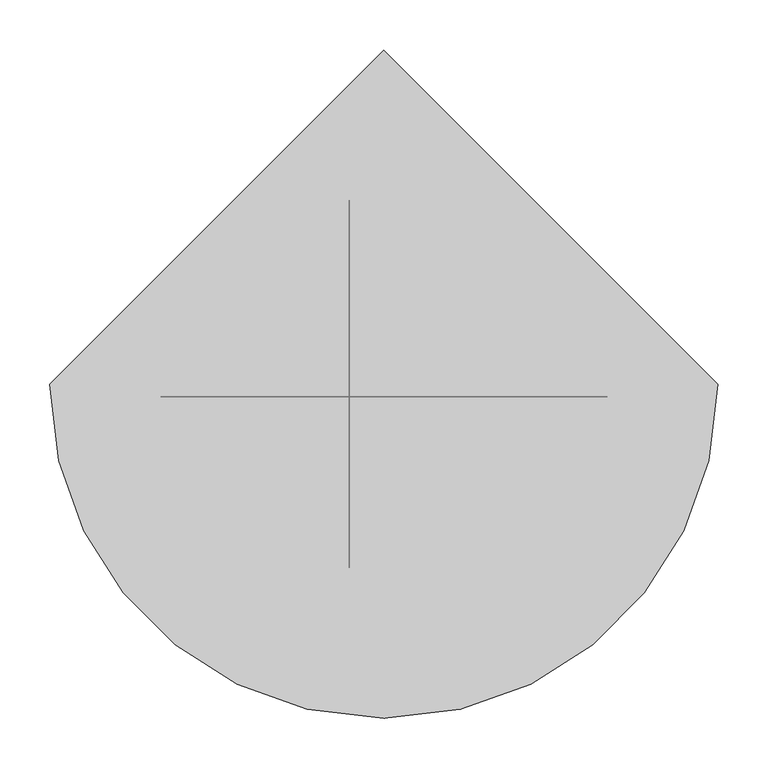
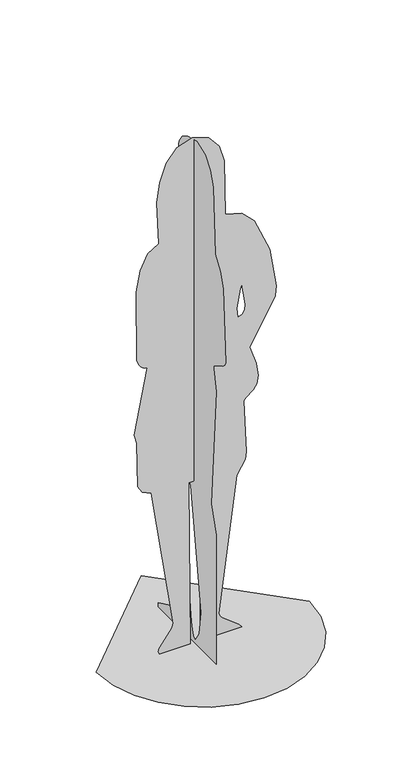
"""IFC4 building model written with IfcOpenShell, lengths in millimetres: proxy geometry, florence 23626 : florence 23626."""

import ifcopenshell
import ifcopenshell.guid

model = None  # the IFC model being written
_history = None  # IfcOwnerHistory: only IFC2X3 demands one
_inside = {}  # id of a spatial element -> (the spatial element, [elements in it])
_under = {}  # id of a project, library or spatial element -> (it, [spatial elements below it])
_declared = {}  # id of a project -> (the project, [libraries it declares])
_typed = {}  # id of a type object -> (the type object, [elements of that type])
_made_of = {}  # id of a material, layer set ... -> (it, [elements and type objects made of it])


def new_model(schema):
    """Start an empty IFC model of exactly this schema.

    Asked for "IFC4X3", IfcOpenShell would pick the latest addendum, in which some entities
    have other attributes; the version numbers below select the first issue.
    IFC2X3 requires an IfcOwnerHistory on every rooted entity: one is made here for all.
    """
    global model, _history
    if schema == "IFC4X3":
        model = ifcopenshell.file(schema_version=(4, 3, 0, 0))
    else:
        model = ifcopenshell.file(schema=schema)
    _inside.clear()
    _under.clear()
    _declared.clear()
    _typed.clear()
    _made_of.clear()
    _history = None
    if model.schema == "IFC2X3":
        org = make("IfcOrganization", Name="unknown")
        user = make(
            "IfcPersonAndOrganization",
            ThePerson=make("IfcPerson", FamilyName="unknown"),
            TheOrganization=org,
        )
        app = make(
            "IfcApplication",
            ApplicationDeveloper=org,
            Version="unknown",
            ApplicationFullName="unknown",
            ApplicationIdentifier="unknown",
        )
        _history = make(
            "IfcOwnerHistory",
            OwningUser=user,
            OwningApplication=app,
            ChangeAction="ADDED",
            CreationDate=0,
        )
    return model


def make(cls, **values):
    """One entity of the class cls with the attributes given. An attribute that is None is left unset."""
    return model.create_entity(
        cls, **{name: value for name, value in values.items() if value is not None}
    )


def rooted(cls, **values):
    """An entity with a GlobalId (a new one), such as an element, a storey or a relation."""
    return make(cls, GlobalId=ifcopenshell.guid.new(), OwnerHistory=_history, **values)


def si_unit(unit_type, name, prefix=None):
    """IfcSIUnit, for example si_unit("LENGTHUNIT", "METRE", prefix="MILLI")."""
    return make("IfcSIUnit", UnitType=unit_type, Prefix=prefix, Name=name)


def assignment(units):
    """IfcUnitAssignment: the units of a project."""
    return None if units is None else make("IfcUnitAssignment", Units=units)


def point(xyz):
    """IfcCartesianPoint."""
    return None if xyz is None else make("IfcCartesianPoint", Coordinates=xyz)


def direction(xyz):
    """IfcDirection."""
    return None if xyz is None else make("IfcDirection", DirectionRatios=xyz)


def frame(location, z_axis=None, x_axis=None):
    """IfcAxis2Placement3D, a coordinate frame: its origin and axes. An axis left out is left unset."""
    return make(
        "IfcAxis2Placement3D",
        Location=point(location),
        Axis=direction(z_axis),
        RefDirection=direction(x_axis),
    )


def origin():
    """The frame at (0, 0, 0) with its axes left unset."""
    return frame((0.0, 0.0, 0.0))


def place(relative_to, where):
    """IfcLocalPlacement: puts the frame where relative to a parent placement (None: the world)."""
    return make(
        "IfcLocalPlacement", PlacementRelTo=relative_to, RelativePlacement=where
    )


def context(
    kind, dimensions, precision=None, world=None, true_north=None, identifier=None
):
    """IfcGeometricRepresentationContext, for example the 3D "Model" context."""
    return make(
        "IfcGeometricRepresentationContext",
        ContextIdentifier=identifier,
        ContextType=kind,
        CoordinateSpaceDimension=dimensions,
        Precision=precision,
        WorldCoordinateSystem=world,
        TrueNorth=true_north,
    )


def project(units=None, contexts=None):
    """IfcProject with its units and contexts."""
    return rooted(
        "IfcProject",
        Name="project",
        RepresentationContexts=contexts,
        UnitsInContext=assignment(units),
    )


def spatial(cls, under=None, at=None, **own):
    """A site, building, storey or space (cls), placed at a placement, below another one or the project."""
    s = rooted(cls, ObjectPlacement=at, **own)
    if under is not None:
        _under.setdefault(under.id(), (under, []))[1].append(s)
    return s


def point_list(points):
    """IfcCartesianPointList2D or 3D."""
    cls = (
        "IfcCartesianPointList2D" if len(points[0]) == 2 else "IfcCartesianPointList3D"
    )
    return make(cls, CoordList=points)


def triangles(points, corners, closed=None, point_numbers=None):
    """IfcTriangulatedFaceSet: each triangle names its three corners, points numbered from 1."""
    return make(
        "IfcTriangulatedFaceSet",
        Coordinates=point_list(points),
        Closed=closed,
        CoordIndex=corners,
        PnIndex=point_numbers,
    )


def shape(context_of_items, identifier, shape_type, items):
    """IfcShapeRepresentation: the items that make up one representation, for example the "Body"."""
    return make(
        "IfcShapeRepresentation",
        ContextOfItems=context_of_items,
        RepresentationIdentifier=identifier,
        RepresentationType=shape_type,
        Items=items,
    )


def source(mapping_origin, context_of_items, identifier, shape_type, items):
    """IfcRepresentationMap: a shape defined once, which mapped items show again and again."""
    return make(
        "IfcRepresentationMap",
        MappingOrigin=mapping_origin,
        MappedRepresentation=shape(context_of_items, identifier, shape_type, items),
    )


def transform(
    local_origin,
    x_axis=None,
    y_axis=None,
    z_axis=None,
    scale=None,
    scale2=None,
    scale3=None,
    uniform=True,
):
    """IfcCartesianTransformationOperator3D, or its non-uniform kind. x_axis, y_axis, z_axis: its Axis1, 2, 3."""
    if uniform:
        return make(
            "IfcCartesianTransformationOperator3D",
            Axis1=direction(x_axis),
            Axis2=direction(y_axis),
            LocalOrigin=point(local_origin),
            Scale=scale,
            Axis3=direction(z_axis),
        )
    return make(
        "IfcCartesianTransformationOperator3DnonUniform",
        Axis1=direction(x_axis),
        Axis2=direction(y_axis),
        LocalOrigin=point(local_origin),
        Scale=scale,
        Axis3=direction(z_axis),
        Scale2=scale2,
        Scale3=scale3,
    )


def mapped(mapping_source, mapping_target):
    """IfcMappedItem: shows the shape of a source again, moved by a transform."""
    return make(
        "IfcMappedItem", MappingSource=mapping_source, MappingTarget=mapping_target
    )


def made_of(thing, what):
    """Note that an element or type object is made of a material, layer set ...; save() writes the relation."""
    if what is not None:
        _made_of.setdefault(what.id(), (what, []))[1].append(thing)
    return thing


def element(
    cls,
    number,
    at=None,
    inside=None,
    cuts=None,
    type_object=None,
    material=None,
    context=None,
    identifier="Body",
    shape_type=None,
    held_by="IfcProductDefinitionShape",
    body=None,
    shapes=None,
    **own,
):
    """One element of the class cls, such as IfcWall. Its Tag is "e" and its number.

    at: its placement. inside: the storey or other place that contains it. cuts: it is an
    opening in that element (IfcRelVoidsElement). A single representation is given by context,
    identifier, shape_type and body (its items); several are given by shapes. held_by: the class
    of the entity that holds the representations. save() writes the other relations.
    """
    e = rooted(cls, Tag="e%d" % number, ObjectPlacement=at, **own)
    if body is not None:
        shapes = [shape(context, identifier, shape_type, body)]
    if shapes is not None:
        e.Representation = make(held_by, Representations=shapes)
    if inside is not None:
        _inside.setdefault(inside.id(), (inside, []))[1].append(e)
    if cuts is not None:
        rooted(
            "IfcRelVoidsElement", RelatingBuildingElement=cuts, RelatedOpeningElement=e
        )
    if type_object is not None:
        _typed.setdefault(type_object.id(), (type_object, []))[1].append(e)
    return made_of(e, material)


def aggregate(whole, parts):
    """IfcRelAggregates: a whole, such as a stair, and the parts it consists of."""
    return rooted("IfcRelAggregates", RelatingObject=whole, RelatedObjects=parts)


def save(model, path):
    """Write the relations noted so far, then the file.

    IfcRelAggregates (storeys below a building ...), IfcRelContainedInSpatialStructure (elements
    in a storey), IfcRelDefinesByType, IfcRelAssociatesMaterial and IfcRelDeclares: one each for
    every whole, place, type object, material and project.
    """
    for whole, parts in _under.values():
        aggregate(whole, parts)
    for where, things in _inside.values():
        rooted(
            "IfcRelContainedInSpatialStructure",
            RelatedElements=things,
            RelatingStructure=where,
        )
    for kind, things in _typed.values():
        rooted("IfcRelDefinesByType", RelatedObjects=things, RelatingType=kind)
    for what, things in _made_of.values():
        rooted("IfcRelAssociatesMaterial", RelatedObjects=things, RelatingMaterial=what)
    for by, libraries in _declared.values():
        rooted("IfcRelDeclares", RelatingContext=by, RelatedDefinitions=libraries)
    model.write(path)


def entourage_811b314a(model_context):
    return source(origin(), model_context, "Body", "Tessellation", [
        triangles([(-334.1037346, 0.0, 4.67e-05), (-325.2710979, -76.5544842, 4.67e-05), (-300.1159472, -146.8575331, 4.67e-05), (-260.652404, -208.8948801, 4.67e-05), (-208.8949164, -260.6524404, 4.67e-05), (-146.8574967, -300.1158927, 4.67e-05), (-76.5544569, -325.2710979, 4.67e-05), (1.46e-05, -334.1037346, 4.67e-05), (76.5544933, -325.2710979, 4.67e-05), (146.8575512, -300.1159291, 4.67e-05), (208.8949164, -260.652404, 4.67e-05), (260.6524949, -208.8949164, 4.67e-05), (300.1158927, -146.8574877, 4.67e-05), (325.2710979, -76.5544388, 4.67e-05), (334.1037346, 2.92e-05, 4.67e-05), (-4.38e-05, 334.1037346, 4.67e-05), (-34.5734892, 6.9372071, 510.5862036), (-34.5734892, -50.0892028, 122.5869578), (-34.5734892, -40.8605964, 46.3929486), (-34.5734892, -17.156763, 11.3406073), (-34.5734892, -7.4075261, 20.0668393), (-34.5734892, -1.2814486, 37.4286861), (-34.5734892, 2.1839699, 60.406083), (-34.5734892, 46.4924156, 417.5145226), (-34.5734892, 63.110551, 464.5403223), (-34.5734892, 60.1163569, 490.2851171), (-34.5734892, 39.0456045, 536.4626401), (-34.5734892, 31.9761369, 546.3433597), (-34.5734892, -133.6633439, 4.67e-05), (-34.5734892, -131.2494832, 427.6552917), (-34.5734892, -105.4426373, 516.402818), (-34.5734892, -133.6328588, 904.8776161), (-34.5734892, -118.5361059, 971.9484495), (-34.5734892, -119.0608377, 980.9675211), (-34.5734892, -126.7251318, 988.4865389), (-34.5734892, -167.3249611, 1010.3459604), (-34.5734892, -178.3170045, 1020.1671633), (-34.5734892, -183.8333284, 1032.6394398), (-34.5734892, -170.1062048, 1269.4988194), (-34.5734892, -153.1873611, 1316.4971134), (-34.5734892, -126.3409983, 1357.63312), (-34.5734892, -116.7177394, 1573.3395756), (-34.5734892, -100.9946712, 1620.5182365), (-34.5734892, -71.8812047, 1654.7582977), (-34.5734892, -25.3455982, 1670.9407402), (-34.5734892, 21.8030932, 1659.2649994), (-34.5734892, 51.3717599, 1640.0022217), (-34.5734892, 67.2789739, 1615.437006), (-34.5734892, 73.4432687, 1587.8543873), (-34.5734892, 67.1167018, 1429.4550442), (-34.5734892, 62.6127343, 1414.6470818), (-34.5734892, 56.0061109, 1408.6359661), (-34.5734892, 33.6373977, 1398.6160835), (-34.5734892, 16.4514895, 1382.4130028), (-34.5734892, 16.57443, 1366.5170254), (-34.5734892, 23.8043859, 1350.9894848), (-34.5734892, 80.3273189, 1279.6723263), (-34.5734892, 93.6685013, 1248.0555061), (-34.5734892, 101.8995487, 1241.9481754), (-34.5734892, 113.2377919, 1237.3922035), (-34.5734892, 125.7357391, 1233.7834122), (-34.5734892, 137.446089, 1230.5184952), (-34.5734892, 146.4212861, 1226.9929836), (-34.5734892, 150.7139656, 1222.6031353), (-34.5734892, 148.5627251, 1190.0747429), (-34.5734892, 140.3133468, 1099.0845119), (-34.5734892, 138.7466183, 982.8324509), (-34.5734892, 146.619557, 972.1617359), (-34.5734892, 156.6984477, 965.1524254), (-34.5734892, 165.5362258, 953.6295095), (-34.5734892, 177.5235573, 924.4368147), (-34.5734892, 179.6906852, 910.463249), (-34.5734892, 178.6517588, 899.3693041), (-34.5734892, 173.9156017, 893.0032682), (-34.5734892, 141.1934257, 856.8173229), (-34.5734892, 128.9732504, 798.8474602), (-34.5734892, 142.8071262, 650.4621861), (-34.5734892, 172.1241776, 470.1701385), (-34.5734892, 80.165601, 167.8524907), (-34.5734892, 77.6115508, 131.7844796), (-34.5734892, 91.6650172, 75.8743931), (-34.5734892, 102.4533848, 58.8461219), (-34.5734892, 116.402061, 46.2735109), (-34.5734892, 182.1044005, 14.070202), (-34.5734892, 183.8334919, 4.67e-05), (-34.5734892, 53.8343775, 4.67e-05), (-34.5734892, 35.794949, 12.7326758), (-34.5734892, 29.2465433, 15.4350465), (-34.5734892, 27.5086316, 14.8404334), (-34.5734892, 26.3932972, 13.6010264), (-34.5734892, 23.0176312, 4.67e-05), (109.094422, -12.6250356, 1123.2807821), (99.0693254, -12.6250311, 1062.4456146), (101.4219162, -12.6250299, 1032.213085), (115.6876697, -12.6250299, 1036.9381599), (123.3611929, -12.6250311, 1049.3745375), (125.9346278, -12.6250311, 1066.9140919), (115.0699203, -12.6250356, 1135.9380037), (-142.5672426, -12.6249686, 0.0), (-147.4015315, -12.6249686, 9.7557227), (-144.3530348, -12.6249698, 20.3925416), (-104.8322458, -12.6249732, 72.3575519), (-100.9955795, -12.6249732, 87.8546938), (-169.3635721, -12.6250004, 543.0591125), (-197.666423, -12.6250015, 555.605367), (-211.7992995, -12.6250027, 579.9655443), (-214.3378618, -12.6250106, 724.0128565), (-223.4011713, -12.6250129, 753.7932335), (-181.7746968, -12.6250254, 962.6080313), (-189.3708538, -12.6250254, 963.9546787), (-195.9598957, -12.6250254, 967.6156471), (-201.5894939, -12.6250265, 973.0224392), (-206.3073564, -12.6250265, 979.6063396), (-210.1613907, -12.6250265, 986.7992872), (-213.1991414, -12.6250265, 994.0323486), (-215.4684069, -12.6250277, 1000.7370993), (-216.7846056, -12.6250413, 1226.3016014), (-203.5875006, -12.6250458, 1292.6408661), (-180.5929194, -12.6250481, 1341.5987789), (-145.6074186, -12.6250481, 1362.4953232), (-152.3855205, -12.6250572, 1500.6374725), (-142.6606145, -12.6250617, 1563.7968441), (-122.5369881, -12.6250651, 1620.2490669), (-89.3706259, -12.6250685, 1660.8358337), (-40.5175804, -12.6250685, 1676.4), (11.7229672, -12.6250663, 1659.2202347), (43.4644936, -12.6250651, 1619.483416), (59.5218847, -12.6250617, 1565.8930824), (63.2074382, -12.6250504, 1387.0617016), (114.1081058, -12.6250504, 1371.9761398), (153.4324588, -12.625047, 1333.9056438), (202.7227278, -12.6250413, 1222.3996593), (223.4011349, -12.6250333, 1092.6907888), (219.1644204, -12.6250311, 1062.1448336), (139.8069732, -12.625022, 917.9959288), (160.1375546, -12.6250197, 858.7674219), (166.230751, -12.6250163, 817.4798985), (162.0169457, -12.6250152, 790.3472523), (151.4264947, -12.6250129, 773.5839586), (126.837516, -12.6250129, 756.0219492), (120.6997365, -12.6250118, 747.6516026), (128.6617233, -12.6250015, 575.4503403), (125.4421796, -12.6250004, 551.8412436), (98.6847922, -12.6249981, 508.0167383), (41.8823772, -12.6249732, 71.4770234), (45.3586594, -12.6249709, 61.0228059), (53.9452719, -12.6249709, 51.2209333), (105.6092332, -12.6249686, 11.6815362), (114.4082056, -12.6249686, 0.0), (-16.5201387, -12.6249686, 0.0), (-7.7622953, -12.6250004, 535.4248037), (-51.4360047, -12.6250004, 536.7896187), (-47.7041785, -12.6249686, 0.0)], [[15, 16, 1], [14, 15, 1], [14, 1, 2], [13, 14, 2], [13, 2, 3], [13, 3, 4], [12, 13, 4], [11, 12, 4], [11, 4, 5], [11, 5, 6], [11, 6, 7], [11, 7, 8], [11, 8, 9], [11, 9, 10], [91, 29, 20], [91, 20, 21], [19, 20, 29], [84, 85, 86], [83, 84, 86], [82, 83, 86], [91, 21, 22], [90, 91, 22], [18, 19, 29], [18, 29, 30], [18, 30, 31], [17, 18, 31], [89, 90, 22], [28, 17, 31], [81, 82, 86], [81, 86, 87], [81, 87, 88], [89, 22, 23], [88, 89, 23], [81, 88, 23], [80, 81, 23], [79, 80, 23], [79, 23, 24], [79, 24, 25], [78, 79, 25], [78, 25, 26], [78, 26, 27], [77, 78, 27], [77, 27, 28], [77, 28, 31], [76, 77, 31], [76, 31, 32], [75, 76, 32], [75, 32, 33], [74, 75, 33], [74, 33, 34], [73, 74, 34], [72, 73, 34], [71, 72, 34], [70, 71, 34], [69, 70, 34], [68, 69, 34], [67, 68, 34], [66, 67, 34], [66, 34, 35], [65, 66, 35], [65, 35, 36], [65, 36, 37], [65, 37, 38], [65, 38, 39], [64, 65, 39], [63, 64, 39], [62, 63, 39], [61, 62, 39], [60, 61, 39], [59, 60, 39], [58, 59, 39], [57, 58, 39], [57, 39, 40], [57, 40, 41], [56, 57, 41], [55, 56, 41], [54, 55, 41], [53, 54, 41], [53, 41, 42], [52, 53, 42], [51, 52, 42], [50, 51, 42], [50, 42, 43], [50, 43, 44], [50, 44, 45], [50, 45, 46], [49, 50, 46], [49, 46, 47], [49, 47, 48], [148, 149, 150], [147, 148, 150], [146, 147, 150], [145, 146, 150], [145, 150, 151], [144, 145, 151], [94, 104, 105], [94, 105, 106], [94, 106, 107], [94, 107, 108], [94, 108, 109], [93, 94, 109], [153, 99, 100], [153, 100, 101], [153, 101, 102], [143, 144, 151], [142, 143, 151], [153, 102, 103], [152, 153, 103], [152, 103, 104], [152, 104, 94], [151, 152, 94], [151, 94, 95], [92, 93, 109], [92, 109, 110], [92, 110, 111], [92, 111, 112], [92, 112, 113], [92, 113, 114], [92, 114, 115], [92, 115, 116], [92, 116, 117], [92, 117, 118], [98, 92, 118], [98, 118, 119], [98, 119, 120], [98, 120, 121], [98, 121, 122], [98, 122, 123], [98, 123, 124], [98, 124, 125], [141, 142, 151], [141, 151, 95], [140, 141, 95], [139, 140, 95], [138, 139, 95], [125, 126, 127], [125, 127, 128], [129, 130, 131], [129, 131, 132], [129, 132, 133], [129, 133, 134], [136, 137, 138], [135, 136, 138], [135, 138, 95], [134, 135, 95], [134, 95, 96], [134, 96, 97], [125, 128, 129], [98, 125, 129], [98, 129, 134], [98, 134, 97]], closed=False),
    ])


if __name__ == "__main__":
    model = new_model("IFC4")
    model_context = context("Model", 3, world=origin())
    ifc_project = project(units=[si_unit("LENGTHUNIT", "METRE", prefix="MILLI")], contexts=[model_context])
    site = spatial("IfcSite", under=ifc_project)
    building = spatial("IfcBuilding", under=site)
    placement = place(None, origin())
    entourage_shape = entourage_811b314a(model_context)
    element("IfcBuildingElementProxy", 1, Name="florence 23626 : florence 23626", ObjectType="florence 23626 : florence 23626", at=placement, inside=building, context=model_context, shape_type="MappedRepresentation", body=[
        mapped(entourage_shape, transform((0.0, 0.0, 0.0), x_axis=(1.0, 0.0, 0.0), y_axis=(0.0, 1.0, 0.0), z_axis=(0.0, 0.0, 1.0))),
    ])
    save(model, "model.ifc")

# Revit data of these elements
# Type "florence 23626 : florence 23626"
#   built-in parameter 1005195 = "RPC-8-G3AF-G2XX-UFB5-G"
#   Height = 0
